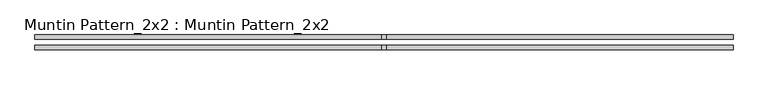
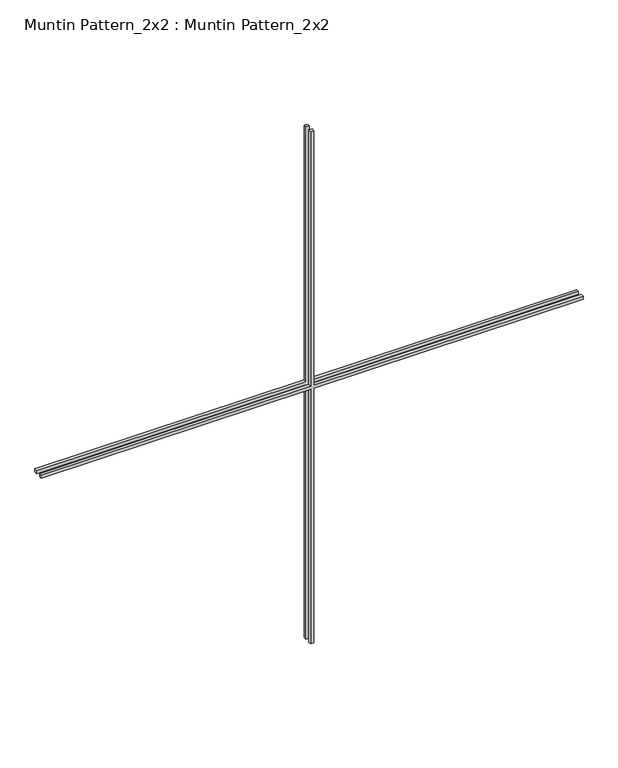
"""IFC4 building model written with IfcOpenShell, lengths in millimetres: proxy geometry, Muntin Pattern_2x2 : Muntin Pattern_2x2."""

from ifc_helpers import new_model, si_unit, frame, origin, place, context, project, spatial, polyline, outline, extrude, source, transform, mapped, element, save


def muntin_pattern_2x2_muntin_pattern_2x2_f50e86f9(model_context):
    return source(origin(), model_context, "Body", "SweptSolid", [
        extrude(outline(polyline([(1068.25, -6.35), (1068.25, -1061.9), (1055.55, -1061.9), (1055.55, -6.35), (0.0, -6.35), (0.0, 6.35), (1055.55, 6.35), (1055.55, 1061.9), (1068.25, 1061.9), (1068.25, 6.35), (2123.8, 6.35), (2123.8, -6.35), (1068.25, -6.35)])), frame((0.0, 9.525, 0.0), z_axis=(0.0, 1.0, 0.0), x_axis=(0.0, 0.0, 1.0)), (0.0, 0.0, 1.0), 12.7),
        extrude(outline(polyline([(1068.25, -6.35), (1068.25, -1061.9), (1055.55, -1061.9), (1055.55, -6.35), (0.0, -6.35), (0.0, 6.35), (1055.55, 6.35), (1055.55, 1061.9), (1068.25, 1061.9), (1068.25, 6.35), (2123.8, 6.35), (2123.8, -6.35), (1068.25, -6.35)])), frame((0.0, -22.225, 0.0), z_axis=(0.0, 1.0, 0.0), x_axis=(0.0, 0.0, 1.0)), (0.0, 0.0, 1.0), 12.7),
    ])


if __name__ == "__main__":
    model = new_model("IFC4")
    model_context = context("Model", 3, world=origin())
    ifc_project = project(units=[si_unit("LENGTHUNIT", "METRE", prefix="MILLI")], contexts=[model_context])
    site = spatial("IfcSite", under=ifc_project)
    building = spatial("IfcBuilding", under=site)
    placement = place(None, origin())
    muntin_pattern_2x2_muntin_pattern_2x2_shape = muntin_pattern_2x2_muntin_pattern_2x2_f50e86f9(model_context)
    element("IfcBuildingElementProxy", 1, Name="Muntin Pattern_2x2 : Muntin Pattern_2x2", ObjectType="Muntin Pattern_2x2 : Muntin Pattern_2x2", at=placement, inside=building, context=model_context, shape_type="MappedRepresentation", body=[
        mapped(muntin_pattern_2x2_muntin_pattern_2x2_shape, transform((0.0, 0.0, 0.0), x_axis=(1.0, 0.0, 0.0), y_axis=(0.0, 1.0, 0.0), z_axis=(0.0, 0.0, 1.0))),
    ])
    save(model, "model.ifc")

# Revit data of these elements
# Type "Muntin Pattern_2x2 : Muntin Pattern_2x2"
#   Width [instance default] = 1.2192 m
#   Thickness = 0.0127 m
#   Height [instance default] = 1.2192 m
#   Distance = 0.01905 m
#   Interior Material [instance default] = none
#   Exterior Material [instance default] = none
#   Default Elevation = 0
# Element 1 (IfcBuildingElementProxy, "Muntin Pattern_2x2 : Muntin Pattern_2x2")
#   Width = 2.1238 m
#   Height = 2.1238 m
#   Interior Material = Wood - Stained
#   Exterior Material = Clad - White
#   Materials on its faces: "Clad - White", "Wood - Stained"
# Materials
#   "Clad - White": class "Wood", colour RGB 242 242 238, transparency 0, Cost = 0
#   "Wood - Stained": class "Wood", colour RGB 227 170 128, transparency 0, Cost = 0
